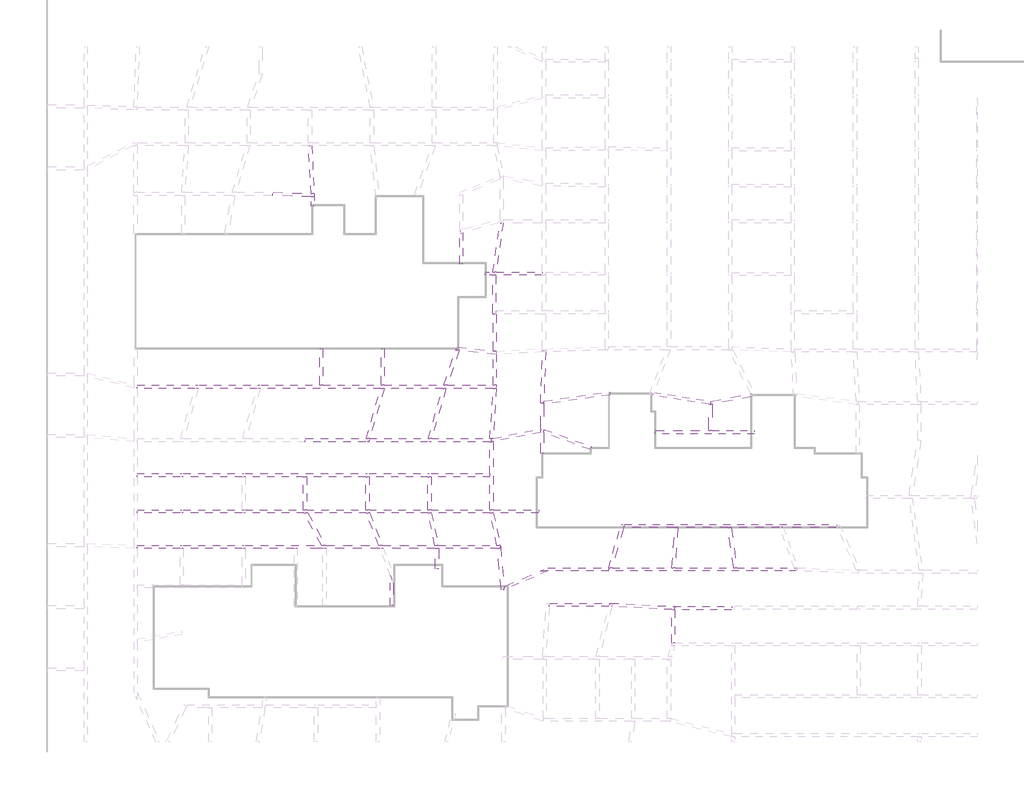
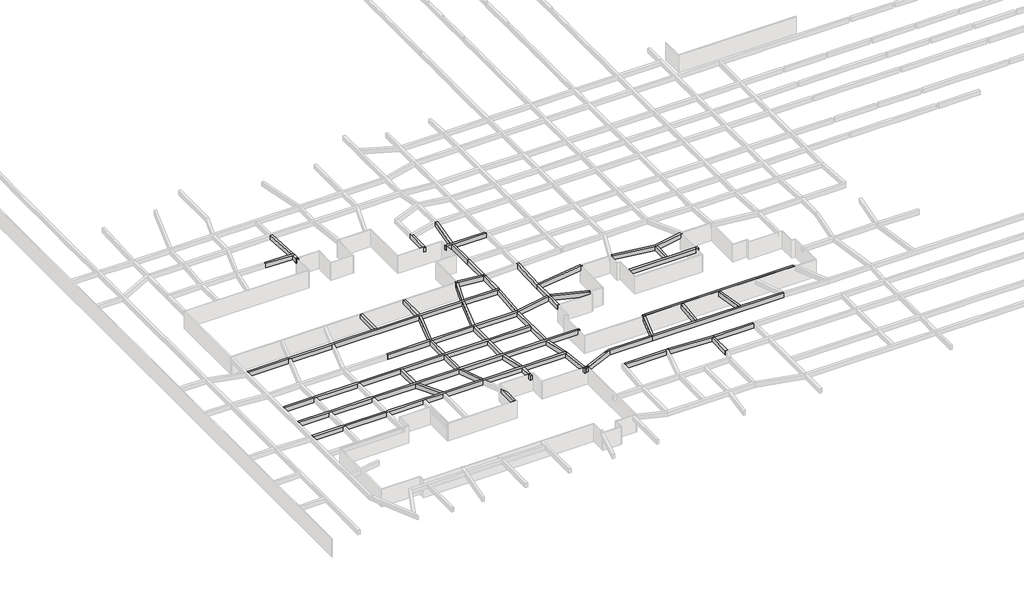
# One storey, part 19 of 45: 53 beams.
"""IFC4 building model written with IfcOpenShell, lengths in millimetres."""

from ifc_helpers import new_model, si_unit, frame, origin, place, context, project, spatial, polyline, outline, extrude, faceted_brep, element, save

model = new_model("IFC4")

# Units and contexts
model_context = context("Model", 3, world=origin())
ifc_project = project(units=[si_unit("LENGTHUNIT", "METRE", prefix="MILLI")], contexts=[model_context])

# Site, building, storey
site = spatial("IfcSite", under=ifc_project)
building = spatial("IfcBuilding", under=site)
storey = spatial("IfcBuildingStorey", under=building, Name="户型图", Elevation=0.0)

# Beams
placement = place(None, origin())
element("IfcBeam", 1, ObjectType="混凝土 - 矩形梁 : KL_beam", at=placement, inside=storey, context=model_context, shape_type="Brep", body=[
    faceted_brep([(-121416.9966498, -9324.8832397, 3300.0), (-121818.2799848, -9310.8701169, 3300.0), (-126600.5942652, -9143.8680223, 3300.0), (-126607.5762912, -9543.8680223, 3300.0), (-121807.1214928, -9711.5035977, 3300.0), (-121430.9564485, -9724.6395705, 3300.0), (-121423.7596296, -9518.5496432, 3300.0), (-126607.5762912, -9543.8680223, 2500.0), (-121807.1214928, -9711.5035977, 2500.0), (-121430.9564485, -9724.6395705, 2500.0), (-126600.5942652, -9143.8680223, 2500.0), (-121818.2799848, -9310.8701169, 2500.0), (-121416.9966498, -9324.8832397, 2500.0), (-121423.7596296, -9518.5496432, 2500.0)], [[[0, 1, 2, 3, 4, 5, 6]], [[5, 4, 3, 7, 8, 9]], [[9, 8, 7, 10, 11, 12, 13]], [[2, 1, 0, 12, 11, 10]], [[2, 10, 7, 3]], [[0, 6, 5, 9, 13, 12]]]),
])
element("IfcBeam", 2, ObjectType="混凝土 - 矩形梁 : KL_beam", at=placement, inside=storey, context=model_context, shape_type="SweptSolid", body=[
    extrude(outline(polyline([(-121416.9966498, -9324.8832397), (-121818.2799848, -9310.8701169), (-122132.953931, -3306.533538), (-121732.4049926, -3306.533538), (-121416.9966498, -9324.8832397)])), frame((0.0, 0.0, 2500.0), z_axis=(0.0, 0.0, 1.0), x_axis=(1.0, 0.0, 0.0)), (0.0, 0.0, 1.0), 800.0),
])
element("IfcBeam", 3, ObjectType="混凝土 - 矩形梁 : KL_beam", at=placement, inside=storey, context=model_context, shape_type="SweptSolid", body=[
    extrude(outline(polyline([(-121407.1214928, -10918.5496432), (-121807.1214928, -10918.5496432), (-121807.1214928, -9711.5035977), (-121430.9564485, -9724.6395705), (-121423.7596296, -9518.5496432), (-121407.1214928, -9518.5496432), (-121407.1214928, -10918.5496432)])), frame((0.0, 0.0, 2500.0), z_axis=(0.0, 0.0, 1.0), x_axis=(1.0, 0.0, 0.0)), (0.0, 0.0, 1.0), 800.0),
])
element("IfcBeam", 4, ObjectType="混凝土 - 矩形梁 : KL_beam", at=placement, inside=storey, context=model_context, shape_type="SweptSolid", body=[
    extrude(outline(polyline([(-102709.6713464, -18172.9434458), (-103109.6713464, -18172.9434458), (-103109.6713464, -13919.4780482), (-103006.1437284, -14305.8483787), (-102709.6713464, -14226.4088434), (-102709.6713464, -18172.9434458)])), frame((0.0, 0.0, 2500.0), z_axis=(0.0, 0.0, 1.0), x_axis=(1.0, 0.0, 0.0)), (0.0, 0.0, 1.0), 800.0),
])
element("IfcBeam", 5, ObjectType="混凝土 - 矩形梁 : KL_beam", at=placement, inside=storey, context=model_context, shape_type="Brep", body=[
    faceted_brep([(-99891.6040575, -19606.533538, 3300.0), (-99891.6040575, -19206.533538, 3300.0), (-99891.6040575, -19206.533538, 2500.0), (-99891.6040575, -19606.533538, 2500.0), (-98951.6884215, -19606.533538, 3300.0), (-98551.6884215, -19606.533538, 3300.0), (-92691.6701424, -19606.533538, 3300.0), (-92691.6701424, -19206.533538, 3300.0), (-98521.6747222, -19206.533538, 3300.0), (-98925.6057512, -19206.533538, 3300.0), (-92691.6701424, -19206.533538, 2500.0), (-98521.6747222, -19206.533538, 2500.0), (-98925.6057512, -19206.533538, 2500.0), (-92691.6701424, -19606.533538, 2500.0), (-98551.6884215, -19606.533538, 2500.0), (-98951.6884215, -19606.533538, 2500.0)], [[[0, 1, 2, 3]], [[1, 0, 4, 5, 6, 7, 8, 9]], [[2, 1, 9, 8, 7, 10, 11, 12]], [[3, 2, 12, 11, 10, 13, 14, 15]], [[0, 3, 15, 14, 13, 6, 5, 4]], [[7, 6, 13, 10]]]),
])
element("IfcBeam", 6, ObjectType="混凝土 - 矩形梁 : KL_beam", at=placement, inside=storey, context=model_context, shape_type="SweptSolid", body=[
    extrude(outline(polyline([(-98521.6747222, -19206.533538), (-98925.6057512, -19206.533538), (-98050.230566, -12977.9154491), (-98010.1601463, -12967.1786125), (-98010.1601463, -13006.533538), (-97650.3215471, -13006.533538), (-98521.6747222, -19206.533538)])), frame((0.0, 0.0, 2500.0), z_axis=(0.0, 0.0, 1.0), x_axis=(1.0, 0.0, 0.0)), (0.0, 0.0, 1.0), 800.0),
])
element("IfcBeam", 7, ObjectType="混凝土 - 矩形梁 : KL_beam", at=placement, inside=storey, context=model_context, shape_type="Brep", body=[
    faceted_brep([(-98951.6884215, -24466.2432363, 3300.0), (-98889.6882512, -24466.2432363, 3300.0), (-98551.6884215, -24466.2432363, 3300.0), (-98551.6884215, -24066.2432363, 3300.0), (-98551.6884215, -19606.533538, 3300.0), (-98951.6884215, -19606.533538, 3300.0), (-98951.6884215, -24466.2432363, 2500.0), (-98951.6884215, -19606.533538, 2500.0), (-98551.6884215, -24466.2432363, 2500.0), (-98889.6882512, -24466.2432363, 2500.0), (-98551.6884215, -19606.533538, 2500.0), (-98551.6884215, -24066.2432363, 2500.0)], [[[0, 1, 2, 3, 4, 5]], [[6, 0, 5, 7]], [[8, 9, 6, 7, 10, 11]], [[2, 8, 11, 10, 4, 3]], [[5, 4, 10, 7]], [[2, 1, 0, 6, 9, 8]]]),
])
element("IfcBeam", 8, ObjectType="混凝土 - 矩形梁 : KL_beam", at=placement, inside=storey, context=model_context, shape_type="Brep", body=[
    faceted_brep([(-92521.8746508, -35665.7137076, 3300.0), (-92513.6781652, -35430.9970723, 3300.0), (-92298.1056102, -29257.806784, 3300.0), (-92291.5379725, -29069.7342493, 3300.0), (-92691.5379725, -29062.7522233, 3300.0), (-92698.9743886, -29275.7033162, 3300.0), (-92921.8746508, -35658.7316817, 3300.0), (-92691.5379725, -29062.7522233, 2500.0), (-92698.9743886, -29275.7033162, 2500.0), (-92921.8746508, -35658.7316817, 2500.0), (-92291.5379725, -29069.7342493, 2500.0), (-92298.1056102, -29257.806784, 2500.0), (-92513.6781652, -35430.9970723, 2500.0), (-92521.8746508, -35665.7137076, 2500.0)], [[[0, 1, 2, 3, 4, 5, 6]], [[6, 5, 4, 7, 8, 9]], [[9, 8, 7, 10, 11, 12, 13]], [[3, 2, 1, 0, 13, 12, 11, 10]], [[3, 10, 7, 4]], [[0, 6, 9, 13]]]),
])
element("IfcBeam", 9, ObjectType="混凝土 - 矩形梁 : KL_beam", at=placement, inside=storey, context=model_context, shape_type="Brep", body=[
    faceted_brep([(-92521.8746508, -42062.2226947, 3300.0), (-92921.8746508, -42062.2226947, 3300.0), (-92921.8746508, -42062.2226947, 2500.0), (-92521.8746508, -42062.2226947, 2500.0), (-92521.8746508, -39413.7176752, 3300.0), (-92521.8746508, -38987.7193621, 3300.0), (-92521.8746508, -35836.0800422, 3300.0), (-92521.8746508, -35665.7137076, 3300.0), (-92921.8746508, -35658.7316817, 3300.0), (-92921.8746508, -38962.5802329, 3300.0), (-92921.8746508, -39370.0669109, 3300.0), (-92921.8746508, -35658.7316817, 2500.0), (-92921.8746508, -38962.5802329, 2500.0), (-92921.8746508, -39370.0669109, 2500.0), (-92521.8746508, -35665.7137076, 2500.0), (-92521.8746508, -35836.0800422, 2500.0), (-92521.8746508, -38987.7193621, 2500.0), (-92521.8746508, -39413.7176752, 2500.0)], [[[0, 1, 2, 3]], [[1, 0, 4, 5, 6, 7, 8, 9, 10]], [[2, 1, 10, 9, 8, 11, 12, 13]], [[3, 2, 13, 12, 11, 14, 15, 16, 17]], [[0, 3, 17, 16, 15, 14, 7, 6, 5, 4]], [[7, 14, 11, 8]]]),
])
element("IfcBeam", 10, ObjectType="混凝土 - 矩形梁 : KL_beam", at=placement, inside=storey, context=model_context, shape_type="Brep", body=[
    faceted_brep([(-98501.9396833, -33842.9557231, 3300.0), (-98501.9396833, -33442.9557231, 3300.0), (-98889.6882512, -33442.9557231, 3300.0), (-104704.5181871, -33442.9557231, 3300.0), (-105128.1844509, -33442.9557231, 3300.0), (-112586.1473381, -33442.9557231, 3300.0), (-112986.1473381, -33442.9557231, 3300.0), (-120315.2422867, -33442.9557231, 3300.0), (-120715.2422867, -33442.9557231, 3300.0), (-128093.2030313, -33442.9557231, 3300.0), (-128509.3228056, -33442.9557231, 3300.0), (-135893.2030313, -33442.9557231, 3300.0), (-136309.3228056, -33442.9557231, 3300.0), (-143687.6160394, -33442.9557231, 3300.0), (-143687.6160394, -33842.9557231, 3300.0), (-136424.0209599, -33842.9557231, 3300.0), (-136007.9011856, -33842.9557231, 3300.0), (-128624.0209599, -33842.9557231, 3300.0), (-128207.9011856, -33842.9557231, 3300.0), (-113051.6472072, -33842.9557231, 3300.0), (-112635.5274329, -33842.9557231, 3300.0), (-105251.569135, -33842.9557231, 3300.0), (-104835.4493606, -33842.9557231, 3300.0), (-98902.739144, -33842.9557231, 3300.0), (-98501.9396833, -33442.9557231, 2500.0), (-98889.6882512, -33442.9557231, 2500.0), (-104704.5181871, -33442.9557231, 2500.0), (-105128.1844509, -33442.9557231, 2500.0), (-112586.1473381, -33442.9557231, 2500.0), (-112986.1473381, -33442.9557231, 2500.0), (-120315.2422867, -33442.9557231, 2500.0), (-120715.2422867, -33442.9557231, 2500.0), (-128093.2030313, -33442.9557231, 2500.0), (-128509.3228056, -33442.9557231, 2500.0), (-135893.2030313, -33442.9557231, 2500.0), (-136309.3228056, -33442.9557231, 2500.0), (-143687.6160394, -33442.9557231, 2500.0), (-98501.9396833, -33842.9557231, 2500.0), (-98902.739144, -33842.9557231, 2500.0), (-104835.4493606, -33842.9557231, 2500.0), (-105251.569135, -33842.9557231, 2500.0), (-112635.5274329, -33842.9557231, 2500.0), (-113051.6472072, -33842.9557231, 2500.0), (-128207.9011856, -33842.9557231, 2500.0), (-128624.0209599, -33842.9557231, 2500.0), (-136007.9011856, -33842.9557231, 2500.0), (-136424.0209599, -33842.9557231, 2500.0), (-143687.6160394, -33842.9557231, 2500.0)], [[[0, 1, 2, 3, 4, 5, 6, 7, 8, 9, 10, 11, 12, 13, 14, 15, 16, 17, 18, 19, 20, 21, 22, 23]], [[1, 24, 25, 26, 27, 28, 29, 30, 31, 32, 33, 34, 35, 36, 13, 12, 11, 10, 9, 8, 7, 6, 5, 4, 3, 2]], [[24, 37, 38, 39, 40, 41, 42, 43, 44, 45, 46, 47, 36, 35, 34, 33, 32, 31, 30, 29, 28, 27, 26, 25]], [[37, 0, 23, 22, 21, 20, 19, 18, 17, 16, 15, 14, 47, 46, 45, 44, 43, 42, 41, 40, 39, 38]], [[14, 13, 36, 47]], [[0, 37, 24, 1]]]),
])
element("IfcBeam", 11, ObjectType="混凝土 - 矩形梁 : KL_beam", at=placement, inside=storey, context=model_context, shape_type="Brep", body=[
    faceted_brep([(-122515.2422867, -40170.1922876, 3300.0), (-122515.2422867, -40570.1922876, 3300.0), (-114915.2422867, -40570.1922876, 3300.0), (-114564.5314767, -40570.1922876, 3300.0), (-114449.8333224, -40170.1922876, 3300.0), (-114865.9530967, -40170.1922876, 3300.0), (-122515.2422867, -40570.1922876, 2500.0), (-114915.2422867, -40570.1922876, 2500.0), (-114564.5314767, -40570.1922876, 2500.0), (-122515.2422867, -40170.1922876, 2500.0), (-114865.9530967, -40170.1922876, 2500.0), (-114449.8333224, -40170.1922876, 2500.0)], [[[0, 1, 2, 3, 4, 5]], [[1, 6, 7, 8, 3, 2]], [[6, 9, 10, 11, 8, 7]], [[9, 0, 5, 4, 11, 10]], [[0, 9, 6, 1]], [[4, 3, 8, 11]]]),
])
element("IfcBeam", 12, ObjectType="混凝土 - 矩形梁 : KL_beam", at=placement, inside=storey, context=model_context, shape_type="Brep", body=[
    faceted_brep([(-99095.9844771, -40570.1922876, 3300.0), (-99134.5000963, -40170.1922876, 3300.0), (-99302.9736319, -40170.1922876, 3300.0), (-106649.7552501, -40170.1922876, 3300.0), (-107065.8750244, -40170.1922876, 3300.0), (-114449.8333224, -40170.1922876, 3300.0), (-114564.5314767, -40570.1922876, 3300.0), (-114515.2422867, -40570.1922876, 3300.0), (-107115.2422867, -40570.1922876, 3300.0), (-106715.2422867, -40570.1922876, 3300.0), (-99315.2422867, -40570.1922876, 3300.0), (-99095.9844771, -40570.1922876, 2500.0), (-114564.5314767, -40570.1922876, 2500.0), (-114515.2422867, -40570.1922876, 2500.0), (-107115.2422867, -40570.1922876, 2500.0), (-106715.2422867, -40570.1922876, 2500.0), (-99315.2422867, -40570.1922876, 2500.0), (-99134.5000963, -40170.1922876, 2500.0), (-114449.8333224, -40170.1922876, 2500.0), (-107065.8750244, -40170.1922876, 2500.0), (-106649.7552501, -40170.1922876, 2500.0), (-99302.9736319, -40170.1922876, 2500.0)], [[[0, 1, 2, 3, 4, 5, 6, 7, 8, 9, 10]], [[11, 0, 10, 9, 8, 7, 6, 12, 13, 14, 15, 16]], [[17, 11, 16, 15, 14, 13, 12, 18, 19, 20, 21]], [[1, 17, 21, 20, 19, 18, 5, 4, 3, 2]], [[1, 0, 11, 17]], [[6, 5, 18, 12]]]),
])
element("IfcBeam", 13, ObjectType="混凝土 - 矩形梁 : KL_beam", at=placement, inside=storey, context=model_context, shape_type="Brep", body=[
    faceted_brep([(-99134.5000963, -40170.1922876, 3300.0), (-99095.9844771, -40570.1922876, 3300.0), (-98915.2422867, -40535.0595648, 3300.0), (-92921.8746508, -39370.0669109, 3300.0), (-92921.8746508, -38962.5802329, 3300.0), (-98899.2820038, -40124.4705221, 3300.0), (-99095.9844771, -40570.1922876, 2500.0), (-98915.2422867, -40535.0595648, 2500.0), (-92921.8746508, -39370.0669109, 2500.0), (-99134.5000963, -40170.1922876, 2500.0), (-98899.2820038, -40124.4705221, 2500.0), (-92921.8746508, -38962.5802329, 2500.0)], [[[0, 1, 2, 3, 4, 5]], [[1, 6, 7, 8, 3, 2]], [[6, 9, 10, 11, 8, 7]], [[9, 0, 5, 4, 11, 10]], [[0, 9, 6, 1]], [[4, 3, 8, 11]]]),
])
element("IfcBeam", 14, ObjectType="混凝土 - 矩形梁 : KL_beam", at=placement, inside=storey, context=model_context, shape_type="Brep", body=[
    faceted_brep([(-143687.6160394, -44584.7380181, 3300.0), (-143687.6160394, -44984.7380181, 3300.0), (-138287.6160394, -44984.7380181, 3300.0), (-137887.6160394, -44984.7380181, 3300.0), (-130487.6160394, -44984.7380181, 3300.0), (-130087.6160394, -44984.7380181, 3300.0), (-122787.6160394, -44984.7380181, 3300.0), (-122387.6160394, -44984.7380181, 3300.0), (-114915.2422867, -44984.7380181, 3300.0), (-114515.2422867, -44984.7380181, 3300.0), (-107115.2422867, -44984.7380181, 3300.0), (-106715.2422867, -44984.7380181, 3300.0), (-99315.2422867, -44984.7380181, 3300.0), (-99315.2422867, -44584.7380181, 3300.0), (-106715.2422867, -44584.7380181, 3300.0), (-107115.2422867, -44584.7380181, 3300.0), (-114515.2422867, -44584.7380181, 3300.0), (-114915.2422867, -44584.7380181, 3300.0), (-130087.6160394, -44584.7380181, 3300.0), (-130487.6160394, -44584.7380181, 3300.0), (-137887.6160394, -44584.7380181, 3300.0), (-138287.6160394, -44584.7380181, 3300.0), (-143687.6160394, -44984.7380181, 2500.0), (-138287.6160394, -44984.7380181, 2500.0), (-137887.6160394, -44984.7380181, 2500.0), (-130487.6160394, -44984.7380181, 2500.0), (-130087.6160394, -44984.7380181, 2500.0), (-122787.6160394, -44984.7380181, 2500.0), (-122387.6160394, -44984.7380181, 2500.0), (-114915.2422867, -44984.7380181, 2500.0), (-114515.2422867, -44984.7380181, 2500.0), (-107115.2422867, -44984.7380181, 2500.0), (-106715.2422867, -44984.7380181, 2500.0), (-99315.2422867, -44984.7380181, 2500.0), (-143687.6160394, -44584.7380181, 2500.0), (-138287.6160394, -44584.7380181, 2500.0), (-137887.6160394, -44584.7380181, 2500.0), (-130487.6160394, -44584.7380181, 2500.0), (-130087.6160394, -44584.7380181, 2500.0), (-114915.2422867, -44584.7380181, 2500.0), (-114515.2422867, -44584.7380181, 2500.0), (-107115.2422867, -44584.7380181, 2500.0), (-106715.2422867, -44584.7380181, 2500.0), (-99315.2422867, -44584.7380181, 2500.0)], [[[0, 1, 2, 3, 4, 5, 6, 7, 8, 9, 10, 11, 12, 13, 14, 15, 16, 17, 18, 19, 20, 21]], [[1, 22, 23, 24, 25, 26, 27, 28, 29, 30, 31, 32, 33, 12, 11, 10, 9, 8, 7, 6, 5, 4, 3, 2]], [[22, 34, 35, 36, 37, 38, 39, 40, 41, 42, 43, 33, 32, 31, 30, 29, 28, 27, 26, 25, 24, 23]], [[34, 0, 21, 20, 19, 18, 17, 16, 15, 14, 13, 43, 42, 41, 40, 39, 38, 37, 36, 35]], [[1, 0, 34, 22]], [[13, 12, 33, 43]]]),
])
element("IfcBeam", 15, ObjectType="混凝土 - 矩形梁 : KL_beam", at=placement, inside=storey, context=model_context, shape_type="Brep", body=[
    faceted_brep([(-93173.130842, -49149.7368283, 3300.0), (-93173.130842, -49549.7368283, 3300.0), (-93173.130842, -49549.7368283, 2500.0), (-93173.130842, -49149.7368283, 2500.0), (-98915.2422867, -49149.7368283, 3300.0), (-99315.2422867, -49149.7368283, 3300.0), (-106715.2422867, -49149.7368283, 3300.0), (-107115.2422867, -49149.7368283, 3300.0), (-114515.2422867, -49149.7368283, 3300.0), (-114915.2422867, -49149.7368283, 3300.0), (-122387.6160394, -49149.7368283, 3300.0), (-122787.6160394, -49149.7368283, 3300.0), (-130087.6160394, -49149.7368283, 3300.0), (-130487.6160394, -49149.7368283, 3300.0), (-137887.6160394, -49149.7368283, 3300.0), (-138287.6160394, -49149.7368283, 3300.0), (-143687.6160394, -49149.7368283, 3300.0), (-143687.6160394, -49549.7368283, 3300.0), (-138287.6160394, -49549.7368283, 3300.0), (-137887.6160394, -49549.7368283, 3300.0), (-130487.6160394, -49549.7368283, 3300.0), (-130087.6160394, -49549.7368283, 3300.0), (-122705.4250427, -49549.7368283, 3300.0), (-122248.0834155, -49549.7368283, 3300.0), (-114852.5939636, -49549.7368283, 3300.0), (-114424.1359662, -49549.7368283, 3300.0), (-107077.1990933, -49549.7368283, 3300.0), (-106668.2628554, -49549.7368283, 3300.0), (-99277.1990933, -49549.7368283, 3300.0), (-98868.2628554, -49549.7368283, 3300.0), (-143687.6160394, -49549.7368283, 2500.0), (-138287.6160394, -49549.7368283, 2500.0), (-137887.6160394, -49549.7368283, 2500.0), (-130487.6160394, -49549.7368283, 2500.0), (-130087.6160394, -49549.7368283, 2500.0), (-122705.4250427, -49549.7368283, 2500.0), (-122248.0834155, -49549.7368283, 2500.0), (-114852.5939636, -49549.7368283, 2500.0), (-114424.1359662, -49549.7368283, 2500.0), (-107077.1990933, -49549.7368283, 2500.0), (-106668.2628554, -49549.7368283, 2500.0), (-99277.1990933, -49549.7368283, 2500.0), (-98868.2628554, -49549.7368283, 2500.0), (-143687.6160394, -49149.7368283, 2500.0), (-138287.6160394, -49149.7368283, 2500.0), (-137887.6160394, -49149.7368283, 2500.0), (-130487.6160394, -49149.7368283, 2500.0), (-130087.6160394, -49149.7368283, 2500.0), (-122787.6160394, -49149.7368283, 2500.0), (-122387.6160394, -49149.7368283, 2500.0), (-114915.2422867, -49149.7368283, 2500.0), (-114515.2422867, -49149.7368283, 2500.0), (-107115.2422867, -49149.7368283, 2500.0), (-106715.2422867, -49149.7368283, 2500.0), (-99315.2422867, -49149.7368283, 2500.0), (-98915.2422867, -49149.7368283, 2500.0)], [[[0, 1, 2, 3]], [[1, 0, 4, 5, 6, 7, 8, 9, 10, 11, 12, 13, 14, 15, 16, 17, 18, 19, 20, 21, 22, 23, 24, 25, 26, 27, 28, 29]], [[2, 1, 29, 28, 27, 26, 25, 24, 23, 22, 21, 20, 19, 18, 17, 30, 31, 32, 33, 34, 35, 36, 37, 38, 39, 40, 41, 42]], [[3, 2, 42, 41, 40, 39, 38, 37, 36, 35, 34, 33, 32, 31, 30, 43, 44, 45, 46, 47, 48, 49, 50, 51, 52, 53, 54, 55]], [[0, 3, 55, 54, 53, 52, 51, 50, 49, 48, 47, 46, 45, 44, 43, 16, 15, 14, 13, 12, 11, 10, 9, 8, 7, 6, 5, 4]], [[17, 16, 43, 30]]]),
])
element("IfcBeam", 16, ObjectType="混凝土 - 矩形梁 : KL_beam", at=placement, inside=storey, context=model_context, shape_type="Brep", body=[
    faceted_brep([(-98009.5874144, -53989.4871623, 3300.0), (-98009.5874144, -53589.4871623, 3300.0), (-98418.5236523, -53589.4871623, 3300.0), (-105809.5874144, -53589.4871623, 3300.0), (-106218.5236523, -53589.4871623, 3300.0), (-112873.4211024, -53589.4871623, 3300.0), (-113301.8790999, -53589.4871623, 3300.0), (-120008.8132398, -53589.4871623, 3300.0), (-120466.154867, -53589.4871623, 3300.0), (-130087.6160394, -53589.4871623, 3300.0), (-130487.6160394, -53589.4871623, 3300.0), (-137887.6160394, -53589.4871623, 3300.0), (-138287.6160394, -53589.4871623, 3300.0), (-143687.6160394, -53589.4871623, 3300.0), (-143687.6160394, -53989.4871623, 3300.0), (-138287.6160394, -53989.4871623, 3300.0), (-137887.6160394, -53989.4871623, 3300.0), (-130487.6160394, -53989.4871623, 3300.0), (-130087.6160394, -53989.4871623, 3300.0), (-123926.6222431, -53989.4871623, 3300.0), (-123526.6222431, -53989.4871623, 3300.0), (-120326.6222431, -53989.4871623, 3300.0), (-119926.6222431, -53989.4871623, 3300.0), (-113148.3334859, -53989.4871623, 3300.0), (-112719.8754884, -53989.4871623, 3300.0), (-106171.6416274, -53989.4871623, 3300.0), (-105771.6416274, -53989.4871623, 3300.0), (-98354.8677696, -53989.4871623, 3300.0), (-98009.5874144, -53989.4871623, 2500.0), (-143687.6160394, -53989.4871623, 2500.0), (-138287.6160394, -53989.4871623, 2500.0), (-137887.6160394, -53989.4871623, 2500.0), (-130487.6160394, -53989.4871623, 2500.0), (-130087.6160394, -53989.4871623, 2500.0), (-123926.6222431, -53989.4871623, 2500.0), (-123526.6222431, -53989.4871623, 2500.0), (-120326.6222431, -53989.4871623, 2500.0), (-119926.6222431, -53989.4871623, 2500.0), (-113148.3334859, -53989.4871623, 2500.0), (-112719.8754884, -53989.4871623, 2500.0), (-106171.6416274, -53989.4871623, 2500.0), (-105771.6416274, -53989.4871623, 2500.0), (-98354.8677696, -53989.4871623, 2500.0), (-98009.5874144, -53589.4871623, 2500.0), (-143687.6160394, -53589.4871623, 2500.0), (-138287.6160394, -53589.4871623, 2500.0), (-137887.6160394, -53589.4871623, 2500.0), (-130487.6160394, -53589.4871623, 2500.0), (-130087.6160394, -53589.4871623, 2500.0), (-120466.154867, -53589.4871623, 2500.0), (-120008.8132398, -53589.4871623, 2500.0), (-113301.8790999, -53589.4871623, 2500.0), (-112873.4211024, -53589.4871623, 2500.0), (-106218.5236523, -53589.4871623, 2500.0), (-105809.5874144, -53589.4871623, 2500.0), (-98418.5236523, -53589.4871623, 2500.0)], [[[0, 1, 2, 3, 4, 5, 6, 7, 8, 9, 10, 11, 12, 13, 14, 15, 16, 17, 18, 19, 20, 21, 22, 23, 24, 25, 26, 27]], [[28, 0, 27, 26, 25, 24, 23, 22, 21, 20, 19, 18, 17, 16, 15, 14, 29, 30, 31, 32, 33, 34, 35, 36, 37, 38, 39, 40, 41, 42]], [[43, 28, 42, 41, 40, 39, 38, 37, 36, 35, 34, 33, 32, 31, 30, 29, 44, 45, 46, 47, 48, 49, 50, 51, 52, 53, 54, 55]], [[1, 43, 55, 54, 53, 52, 51, 50, 49, 48, 47, 46, 45, 44, 13, 12, 11, 10, 9, 8, 7, 6, 5, 4, 3, 2]], [[14, 13, 44, 29]], [[1, 0, 28, 43]]]),
])
element("IfcBeam", 17, ObjectType="混凝土 - 矩形梁 : KL_beam", at=placement, inside=storey, context=model_context, shape_type="SweptSolid", body=[
    extrude(outline(polyline([(-114449.8333224, -40170.1922876), (-114865.9530967, -40170.1922876), (-113051.6472072, -33842.9557231), (-112635.5274329, -33842.9557231), (-114449.8333224, -40170.1922876)])), frame((0.0, 0.0, 2500.0), z_axis=(0.0, 0.0, 1.0), x_axis=(1.0, 0.0, 0.0)), (0.0, 0.0, 1.0), 800.0),
])
element("IfcBeam", 18, ObjectType="混凝土 - 矩形梁 : KL_beam", at=placement, inside=storey, context=model_context, shape_type="SweptSolid", body=[
    extrude(outline(polyline([(-122787.6160394, -44984.7380181), (-122387.6160394, -44984.7380181), (-122387.6160394, -49149.7368283), (-122787.6160394, -49149.7368283), (-122787.6160394, -44984.7380181)])), frame((0.0, 0.0, 2500.0), z_axis=(0.0, 0.0, 1.0), x_axis=(1.0, 0.0, 0.0)), (0.0, 0.0, 1.0), 800.0),
])
element("IfcBeam", 19, ObjectType="混凝土 - 矩形梁 : KL_beam", at=placement, inside=storey, context=model_context, shape_type="SweptSolid", body=[
    extrude(outline(polyline([(-122705.4250427, -49549.7368283), (-122248.0834155, -49549.7368283), (-120008.8132398, -53589.4871623), (-120466.154867, -53589.4871623), (-122705.4250427, -49549.7368283)])), frame((0.0, 0.0, 2500.0), z_axis=(0.0, 0.0, 1.0), x_axis=(1.0, 0.0, 0.0)), (0.0, 0.0, 1.0), 800.0),
])
element("IfcBeam", 20, ObjectType="混凝土 - 矩形梁 : KL_beam", at=placement, inside=storey, context=model_context, shape_type="Brep", body=[
    faceted_brep([(-114515.2422867, -40570.1922876, 3300.0), (-114564.5314767, -40570.1922876, 3300.0), (-114915.2422867, -40570.1922876, 3300.0), (-114915.2422867, -44584.7380181, 3300.0), (-114515.2422867, -44584.7380181, 3300.0), (-114915.2422867, -40570.1922876, 2500.0), (-114915.2422867, -44584.7380181, 2500.0), (-114564.5314767, -40570.1922876, 2500.0), (-114515.2422867, -40570.1922876, 2500.0), (-114515.2422867, -44584.7380181, 2500.0)], [[[0, 1, 2, 3, 4]], [[2, 5, 6, 3]], [[5, 7, 8, 9, 6]], [[8, 0, 4, 9]], [[5, 2, 1, 0, 8, 7]], [[4, 3, 6, 9]]]),
    faceted_brep([(-114515.2422867, -49149.7368283, 3300.0), (-114915.2422867, -49149.7368283, 3300.0), (-114915.2422867, -49149.7368283, 2500.0), (-114515.2422867, -49149.7368283, 2500.0), (-114915.2422867, -44984.7380181, 3300.0), (-114515.2422867, -44984.7380181, 3300.0), (-114515.2422867, -44984.7380181, 2500.0), (-114915.2422867, -44984.7380181, 2500.0)], [[[0, 1, 2, 3]], [[4, 5, 6, 7]], [[1, 0, 5, 4]], [[2, 1, 4, 7]], [[3, 2, 7, 6]], [[0, 3, 6, 5]]]),
])
element("IfcBeam", 21, ObjectType="混凝土 - 矩形梁 : KL_beam", at=placement, inside=storey, context=model_context, shape_type="SweptSolid", body=[
    extrude(outline(polyline([(-114852.5939636, -49549.7368283), (-114424.1359662, -49549.7368283), (-112873.4211024, -53589.4871623), (-113301.8790999, -53589.4871623), (-114852.5939636, -49549.7368283)])), frame((0.0, 0.0, 2500.0), z_axis=(0.0, 0.0, 1.0), x_axis=(1.0, 0.0, 0.0)), (0.0, 0.0, 1.0), 800.0),
])
element("IfcBeam", 22, ObjectType="混凝土 - 矩形梁 : KL_beam", at=placement, inside=storey, context=model_context, shape_type="SweptSolid", body=[
    extrude(outline(polyline([(-107115.2422867, -40570.1922876), (-106715.2422867, -40570.1922876), (-106715.2422867, -44584.7380181), (-107115.2422867, -44584.7380181), (-107115.2422867, -40570.1922876)])), frame((0.0, 0.0, 2500.0), z_axis=(0.0, 0.0, 1.0), x_axis=(1.0, 0.0, 0.0)), (0.0, 0.0, 1.0), 800.0),
    extrude(outline(polyline([(-106715.2422867, -49149.7368283), (-107115.2422867, -49149.7368283), (-107115.2422867, -44984.7380181), (-106715.2422867, -44984.7380181), (-106715.2422867, -49149.7368283)])), frame((0.0, 0.0, 2500.0), z_axis=(0.0, 0.0, 1.0), x_axis=(1.0, 0.0, 0.0)), (0.0, 0.0, 1.0), 800.0),
])
element("IfcBeam", 23, ObjectType="混凝土 - 矩形梁 : KL_beam", at=placement, inside=storey, context=model_context, shape_type="SweptSolid", body=[
    extrude(outline(polyline([(-107077.1990933, -49549.7368283), (-106668.2628554, -49549.7368283), (-105809.5874144, -53589.4871623), (-106218.5236523, -53589.4871623), (-107077.1990933, -49549.7368283)])), frame((0.0, 0.0, 2500.0), z_axis=(0.0, 0.0, 1.0), x_axis=(1.0, 0.0, 0.0)), (0.0, 0.0, 1.0), 800.0),
])
element("IfcBeam", 24, ObjectType="混凝土 - 矩形梁 : KL_beam", at=placement, inside=storey, context=model_context, shape_type="Brep", body=[
    faceted_brep([(-99095.9844771, -40570.1922876, 3300.0), (-99315.2422867, -40570.1922876, 3300.0), (-99315.2422867, -44584.7380181, 3300.0), (-99315.2422867, -44984.7380181, 3300.0), (-99315.2422867, -49149.7368283, 3300.0), (-98915.2422867, -49149.7368283, 3300.0), (-98915.2422867, -40535.0595648, 3300.0), (-99315.2422867, -40570.1922876, 2500.0), (-99315.2422867, -44584.7380181, 2500.0), (-99315.2422867, -44984.7380181, 2500.0), (-99315.2422867, -49149.7368283, 2500.0), (-99095.9844771, -40570.1922876, 2500.0), (-98915.2422867, -40535.0595648, 2500.0), (-98915.2422867, -49149.7368283, 2500.0)], [[[0, 1, 2, 3, 4, 5, 6]], [[1, 7, 8, 9, 10, 4, 3, 2]], [[7, 11, 12, 13, 10, 9, 8]], [[12, 6, 5, 13]], [[1, 0, 11, 7]], [[0, 6, 12, 11]], [[5, 4, 10, 13]]]),
])
element("IfcBeam", 25, ObjectType="混凝土 - 矩形梁 : KL_beam", at=placement, inside=storey, context=model_context, shape_type="SweptSolid", body=[
    extrude(outline(polyline([(-98009.5874144, -53589.4871623), (-98418.5236523, -53589.4871623), (-99277.1990933, -49549.7368283), (-98868.2628554, -49549.7368283), (-98009.5874144, -53589.4871623)])), frame((0.0, 0.0, 2500.0), z_axis=(0.0, 0.0, 1.0), x_axis=(1.0, 0.0, 0.0)), (0.0, 0.0, 1.0), 800.0),
])
element("IfcBeam", 26, ObjectType="混凝土 - 矩形梁 : KL_beam", at=placement, inside=storey, context=model_context, shape_type="Brep", body=[
    faceted_brep([(-97497.8255668, -59196.0390677, 3300.0), (-97534.4934161, -58776.9236321, 3300.0), (-97973.4688225, -53759.4117772, 3300.0), (-98009.5874144, -53589.4871623, 3300.0), (-98009.5874144, -53989.4871623, 3300.0), (-98354.8677696, -53989.4871623, 3300.0), (-97896.303446, -59230.9013648, 3300.0), (-97896.303446, -59230.9013648, 2500.0), (-98354.8677696, -53989.4871623, 2500.0), (-97973.4688225, -53759.4117772, 2500.0), (-97534.4934161, -58776.9236321, 2500.0), (-97497.8255668, -59196.0390677, 2500.0), (-98009.5874144, -53989.4871623, 2500.0), (-98009.5874144, -53589.4871623, 2500.0)], [[[0, 1, 2, 3, 4, 5, 6]], [[7, 6, 5, 8]], [[9, 10, 11, 7, 8, 12, 13]], [[2, 1, 0, 11, 10, 9]], [[3, 2, 9, 13]], [[4, 12, 8, 5]], [[12, 4, 3, 13]], [[0, 6, 7, 11]]]),
])
element("IfcBeam", 27, ObjectType="混凝土 - 矩形梁 : KL_beam", at=placement, inside=storey, context=model_context, shape_type="SweptSolid", body=[
    extrude(outline(polyline([(-105771.6416274, -56588.7580318), (-106171.6416274, -56588.7580318), (-106171.6416274, -53989.4871623), (-105771.6416274, -53989.4871623), (-105771.6416274, -56588.7580318)])), frame((0.0, 0.0, 2500.0), z_axis=(0.0, 0.0, 1.0), x_axis=(1.0, 0.0, 0.0)), (0.0, 0.0, 1.0), 800.0),
])
element("IfcBeam", 28, ObjectType="混凝土 - 矩形梁 : KL_beam", at=placement, inside=storey, context=model_context, shape_type="SweptSolid", body=[
    extrude(outline(polyline([(-111449.0790859, -61137.092783), (-111849.0790859, -61137.092783), (-111849.0790859, -57374.1605919), (-111449.0790859, -58416.1962178), (-111449.0790859, -61137.092783)])), frame((0.0, 0.0, 2500.0), z_axis=(0.0, 0.0, 1.0), x_axis=(1.0, 0.0, 0.0)), (0.0, 0.0, 1.0), 800.0),
])
element("IfcBeam", 29, ObjectType="混凝土 - 矩形梁 : KL_beam", at=placement, inside=storey, context=model_context, shape_type="SweptSolid", body=[
    extrude(outline(polyline([(-105251.569135, -33842.9557231), (-104835.4493606, -33842.9557231), (-106649.7552501, -40170.1922876), (-107065.8750244, -40170.1922876), (-105251.569135, -33842.9557231)])), frame((0.0, 0.0, 2500.0), z_axis=(0.0, 0.0, 1.0), x_axis=(1.0, 0.0, 0.0)), (0.0, 0.0, 1.0), 800.0),
])
element("IfcBeam", 30, ObjectType="混凝土 - 矩形梁 : KL_beam", at=placement, inside=storey, context=model_context, shape_type="Brep", body=[
    faceted_brep([(-98476.6373585, -33442.9557231, 3300.0), (-98489.6882512, -33442.9557231, 3300.0), (-98501.9396833, -33442.9557231, 3300.0), (-98501.9396833, -33842.9557231, 3300.0), (-98476.6373585, -33442.9557231, 2500.0), (-98899.2820038, -40124.4705221, 3300.0), (-98899.2820038, -40124.4705221, 2500.0), (-98501.9396833, -33842.9557231, 2500.0), (-98501.9396833, -33442.9557231, 2500.0), (-98489.6882512, -33442.9557231, 2500.0), (-98902.739144, -33842.9557231, 3300.0), (-98902.739144, -33842.9557231, 2500.0), (-99302.9736319, -40170.1922876, 2500.0), (-99302.9736319, -40170.1922876, 3300.0), (-99134.5000963, -40170.1922876, 3300.0), (-99134.5000963, -40170.1922876, 2500.0)], [[[0, 1, 2, 3]], [[4, 0, 3, 5, 6, 7]], [[8, 9, 4, 7]], [[10, 11, 12, 13]], [[0, 4, 9, 8, 2, 1]], [[3, 7, 11, 10]], [[7, 3, 2, 8]], [[3, 10, 13, 14, 5]], [[11, 7, 6, 15, 12]], [[15, 14, 13, 12]], [[14, 15, 6, 5]]]),
])
element("IfcBeam", 31, ObjectType="混凝土 - 矩形梁 : KL_beam", at=placement, inside=storey, context=model_context, shape_type="Brep", body=[
    faceted_brep([(-98489.6882512, -29133.8276372, 3300.0), (-98682.929173, -29142.4547556, 3300.0), (-98889.6882512, -29151.6853834, 3300.0), (-98889.6882512, -33442.9557231, 3300.0), (-98501.9396833, -33442.9557231, 3300.0), (-98489.6882512, -33442.9557231, 3300.0), (-98489.6882512, -29534.2260627, 3300.0), (-98489.6882512, -29133.8276372, 2500.0), (-98489.6882512, -33442.9557231, 2500.0), (-98489.6882512, -29534.2260627, 2500.0), (-98889.6882512, -29151.6853834, 2500.0), (-98682.929173, -29142.4547556, 2500.0), (-98501.9396833, -33442.9557231, 2500.0), (-98889.6882512, -33442.9557231, 2500.0)], [[[0, 1, 2, 3, 4, 5, 6]], [[7, 0, 6, 5, 8, 9]], [[10, 11, 7, 9, 8, 12, 13]], [[13, 3, 2, 10]], [[3, 13, 12, 8, 5, 4]], [[2, 1, 0, 7, 11, 10]]]),
])
element("IfcBeam", 32, ObjectType="混凝土 - 矩形梁 : KL_beam", at=placement, inside=storey, context=model_context, shape_type="SweptSolid", body=[
    extrude(outline(polyline([(-84233.4038798, -34267.2804127), (-84177.7346394, -34663.3876402), (-92521.8746508, -35836.0800422), (-92521.8746508, -35665.7137076), (-92513.6781652, -35430.9970723), (-84233.4038798, -34267.2804127)])), frame((0.0, 0.0, 2500.0), z_axis=(0.0, 0.0, 1.0), x_axis=(1.0, 0.0, 0.0)), (0.0, 0.0, 1.0), 800.0),
])
element("IfcBeam", 33, ObjectType="混凝土 - 矩形梁 : KL_beam", at=placement, inside=storey, context=model_context, shape_type="SweptSolid", body=[
    extrude(outline(polyline([(-86553.285111, -41174.3422368), (-86690.8837939, -41549.9305786), (-92521.8746508, -39413.7176752), (-92521.8746508, -38987.7193621), (-86553.285111, -41174.3422368)])), frame((0.0, 0.0, 2500.0), z_axis=(0.0, 0.0, 1.0), x_axis=(1.0, 0.0, 0.0)), (0.0, 0.0, 1.0), 800.0),
])
element("IfcBeam", 34, ObjectType="混凝土 - 矩形梁 : KL_beam", at=placement, inside=storey, context=model_context, shape_type="Brep", body=[
    faceted_brep([(-60705.9072961, -56839.7832418, 3300.0), (-60698.9252702, -56439.7832418, 3300.0), (-60988.0458845, -56439.7832418, 3300.0), (-68227.1784385, -56439.7832418, 3300.0), (-68631.2189166, -56439.7832418, 3300.0), (-76006.2262167, -56439.7832418, 3300.0), (-76407.2029759, -56439.7832418, 3300.0), (-83937.0073188, -56439.7832418, 3300.0), (-84353.1270932, -56439.7832418, 3300.0), (-84353.1270932, -56839.7832418, 3300.0), (-60705.9072961, -56839.7832418, 2500.0), (-84353.1270932, -56839.7832418, 2500.0), (-60698.9252702, -56439.7832418, 2500.0), (-84353.1270932, -56439.7832418, 2500.0), (-83937.0073188, -56439.7832418, 2500.0), (-76407.2029759, -56439.7832418, 2500.0), (-76006.2262167, -56439.7832418, 2500.0), (-68631.2189166, -56439.7832418, 2500.0), (-68227.1784385, -56439.7832418, 2500.0), (-60988.0458845, -56439.7832418, 2500.0)], [[[0, 1, 2, 3, 4, 5, 6, 7, 8, 9]], [[10, 0, 9, 11]], [[12, 10, 11, 13, 14, 15, 16, 17, 18, 19]], [[1, 12, 19, 18, 17, 16, 15, 14, 13, 8, 7, 6, 5, 4, 3, 2]], [[1, 0, 10, 12]], [[8, 13, 11, 9]]]),
])
element("IfcBeam", 35, ObjectType="混凝土 - 矩形梁 : KL_beam", at=placement, inside=storey, context=model_context, shape_type="SweptSolid", body=[
    extrude(outline(polyline([(-91804.5472216, -60887.8093836), (-84266.1304086, -60887.8093836), (-84365.8616097, -61287.8093836), (-91832.5179464, -61287.8093836), (-91804.5472216, -60887.8093836)])), frame((0.0, 0.0, 2500.0), z_axis=(0.0, 0.0, 1.0), x_axis=(1.0, 0.0, 0.0)), (0.0, 0.0, 1.0), 800.0),
])
element("IfcBeam", 36, ObjectType="混凝土 - 矩形梁 : KL_beam", at=placement, inside=storey, context=model_context, shape_type="Brep", body=[
    faceted_brep([(-84104.636099, -60887.8093836, 3300.0), (-84266.1304086, -60887.8093836, 3300.0), (-83878.0121181, -60984.5781419, 3300.0), (-83953.616158, -61287.8093836, 3300.0), (-83955.6991422, -61296.1637772, 3300.0), (-76420.6999587, -61691.0563513, 3300.0), (-76020.6999587, -61712.019463, 3300.0), (-76020.6999587, -61701.2648408, 3300.0), (-76020.6999587, -61311.4705246, 3300.0), (-76215.436006, -61301.2648408, 3300.0), (-83955.6991422, -61296.1637772, 2500.0), (-76420.6999587, -61691.0563513, 2500.0), (-76020.6999587, -61712.019463, 2500.0), (-84266.1304086, -60887.8093836, 2500.0), (-84104.636099, -60887.8093836, 2500.0), (-76215.436006, -61301.2648408, 2500.0), (-76020.6999587, -61311.4705246, 2500.0), (-76020.6999587, -61701.2648408, 2500.0), (-83953.616158, -61287.8093836, 2500.0), (-83878.0121181, -60984.5781419, 2500.0)], [[[0, 1, 2, 3, 4, 5, 6, 7, 8, 9]], [[4, 10, 11, 12, 6, 5]], [[13, 14, 15, 16, 17, 12, 11, 10, 18, 19]], [[14, 0, 9, 8, 16, 15]], [[1, 0, 14, 13]], [[2, 19, 18, 10, 4, 3]], [[19, 2, 1, 13]], [[8, 7, 6, 12, 17, 16]]]),
])
element("IfcBeam", 37, ObjectType="混凝土 - 矩形梁 : KL_beam", at=placement, inside=storey, context=model_context, shape_type="SweptSolid", body=[
    extrude(outline(polyline([(-76020.6999587, -65862.2662437), (-76420.6999587, -65862.2662437), (-76420.6999587, -61691.0563513), (-76020.6999587, -61712.019463), (-76020.6999587, -65862.2662437)])), frame((0.0, 0.0, 2500.0), z_axis=(0.0, 0.0, 1.0), x_axis=(1.0, 0.0, 0.0)), (0.0, 0.0, 1.0), 800.0),
])
element("IfcBeam", 38, ObjectType="混凝土 - 矩形梁 : KL_beam", at=placement, inside=storey, context=model_context, shape_type="SweptSolid", body=[
    extrude(outline(polyline([(-68900.6999587, -61301.2648408), (-68900.6999587, -61701.2648408), (-76020.6999587, -61701.2648408), (-76020.6999587, -61311.4705246), (-76215.436006, -61301.2648408), (-68900.6999587, -61301.2648408)])), frame((0.0, 0.0, 2500.0), z_axis=(0.0, 0.0, 1.0), x_axis=(1.0, 0.0, 0.0)), (0.0, 0.0, 1.0), 800.0),
])
element("IfcBeam", 39, ObjectType="混凝土 - 矩形梁 : KL_beam", at=placement, inside=storey, context=model_context, shape_type="Brep", body=[
    faceted_brep([(-78831.4278308, -34714.7552327, 3300.0), (-71745.5456794, -35837.0487115, 3300.0), (-71542.0196166, -35869.284073, 3300.0), (-71549.1082718, -35463.17529, 3300.0), (-78684.8781897, -34332.9803653, 3300.0), (-78831.4278308, -34714.7552327, 2500.0), (-71745.5456794, -35837.0487115, 2500.0), (-71542.0196166, -35869.284073, 2500.0), (-78684.8781897, -34332.9803653, 2500.0), (-71549.1082718, -35463.17529, 2500.0)], [[[0, 1, 2, 3, 4]], [[2, 1, 0, 5, 6, 7]], [[7, 6, 5, 8, 9]], [[3, 9, 8, 4]], [[0, 4, 8, 5]], [[3, 2, 7, 9]]]),
])
element("IfcBeam", 40, ObjectType="混凝土 - 矩形梁 : KL_beam", at=placement, inside=storey, context=model_context, shape_type="Brep", body=[
    faceted_brep([(-71542.0196166, -35869.284073, 3300.0), (-71345.5456794, -35831.0934084, 3300.0), (-66326.6265104, -34855.5143488, 3300.0), (-66508.160593, -34483.3143219, 3300.0), (-71549.1082718, -35463.17529, 3300.0), (-71542.0196166, -35869.284073, 2500.0), (-71345.5456794, -35831.0934084, 2500.0), (-66326.6265104, -34855.5143488, 2500.0), (-71549.1082718, -35463.17529, 2500.0), (-66508.160593, -34483.3143219, 2500.0)], [[[0, 1, 2, 3, 4]], [[2, 1, 0, 5, 6, 7]], [[7, 6, 5, 8, 9]], [[8, 4, 3, 9]], [[4, 8, 5, 0]], [[3, 2, 7, 9]]]),
])
element("IfcBeam", 41, ObjectType="混凝土 - 矩形梁 : KL_beam", at=placement, inside=storey, context=model_context, shape_type="SweptSolid", body=[
    extrude(outline(polyline([(-71542.0196166, -35869.284073), (-71345.5456794, -35831.0934084), (-71345.5456794, -39162.7742653), (-71745.5456794, -39162.7742653), (-71745.5456794, -35837.0487115), (-71542.0196166, -35869.284073)])), frame((0.0, 0.0, 2500.0), z_axis=(0.0, 0.0, 1.0), x_axis=(1.0, 0.0, 0.0)), (0.0, 0.0, 1.0), 800.0),
])
element("IfcBeam", 42, ObjectType="混凝土 - 矩形梁 : KL_beam", at=placement, inside=storey, context=model_context, shape_type="Brep", body=[
    faceted_brep([(-66045.5182206, -39162.7742653, 3300.0), (-66045.5182206, -39562.7742653, 3300.0), (-66045.5182206, -39562.7742653, 2500.0), (-66045.5182206, -39162.7742653, 2500.0), (-78524.5182206, -39162.7742653, 3300.0), (-78524.5182206, -39162.7742653, 2500.0), (-78524.5182206, -39562.7742653, 2500.0), (-78524.5182206, -39562.7742653, 3300.0), (-71345.5456794, -39162.7742653, 3300.0), (-71745.5456794, -39162.7742653, 3300.0), (-71745.5456794, -39162.7742653, 2500.0), (-71345.5456794, -39162.7742653, 2500.0)], [[[0, 1, 2, 3]], [[4, 5, 6, 7]], [[1, 0, 8, 9, 4, 7]], [[2, 1, 7, 6]], [[3, 2, 6, 5, 10, 11]], [[0, 3, 11, 10, 5, 4, 9, 8]]]),
])
element("IfcBeam", 43, ObjectType="混凝土 - 矩形梁 : KL_beam", at=placement, inside=storey, context=model_context, shape_type="Brep", body=[
    faceted_brep([(-92043.2067826, -56439.7832418, 3300.0), (-92983.0367828, -56839.7832418, 3300.0), (-91961.6257837, -56839.7832418, 3300.0), (-84353.1270932, -56839.7832418, 3300.0), (-84353.1270932, -56439.7832418, 3300.0), (-92043.2067826, -56439.7832418, 2500.0), (-84353.1270932, -56439.7832418, 2500.0), (-92983.0367828, -56839.7832418, 2500.0), (-84353.1270932, -56839.7832418, 2500.0), (-91961.6257837, -56839.7832418, 2500.0)], [[[0, 1, 2, 3, 4]], [[5, 0, 4, 6]], [[7, 5, 6, 8, 9]], [[1, 7, 9, 8, 3, 2]], [[4, 3, 8, 6]], [[1, 0, 5, 7]]]),
])
element("IfcBeam", 44, ObjectType="混凝土 - 矩形梁 : KL_beam", at=placement, inside=storey, context=model_context, shape_type="SweptSolid", body=[
    extrude(outline(polyline([(-97497.8255668, -59196.0390677), (-97534.4934161, -58776.9236321), (-92983.0367828, -56839.7832418), (-91961.6257837, -56839.7832418), (-97497.8255668, -59196.0390677)])), frame((0.0, 0.0, 2500.0), z_axis=(0.0, 0.0, 1.0), x_axis=(1.0, 0.0, 0.0)), (0.0, 0.0, 1.0), 800.0),
])
element("IfcBeam", 45, ObjectType="混凝土 - 矩形梁 : KL_beam", at=placement, inside=storey, context=model_context, shape_type="Brep", body=[
    faceted_brep([(-82365.8743907, -50960.5915749, 3300.0), (-82781.994165, -50960.5915749, 3300.0), (-84353.1270932, -56439.7832418, 3300.0), (-83937.0073188, -56439.7832418, 3300.0), (-82480.572545, -51360.5915749, 3300.0), (-82365.8743907, -50960.5915749, 2500.0), (-83937.0073188, -56439.7832418, 2500.0), (-82480.572545, -51360.5915749, 2500.0), (-82781.994165, -50960.5915749, 2500.0), (-84353.1270932, -56439.7832418, 2500.0)], [[[0, 1, 2, 3, 4]], [[5, 0, 4, 3, 6, 7]], [[8, 5, 7, 6, 9]], [[1, 8, 9, 2]], [[3, 2, 9, 6]], [[1, 0, 5, 8]]]),
])
element("IfcBeam", 46, ObjectType="混凝土 - 矩形梁 : KL_beam", at=placement, inside=storey, context=model_context, shape_type="SweptSolid", body=[
    extrude(outline(polyline([(-76006.2262167, -56439.7832418), (-76407.2029759, -56439.7832418), (-76052.0312954, -51360.5915749), (-75651.0545362, -51360.5915749), (-76006.2262167, -56439.7832418)])), frame((0.0, 0.0, 2500.0), z_axis=(0.0, 0.0, 1.0), x_axis=(1.0, 0.0, 0.0)), (0.0, 0.0, 1.0), 800.0),
])
element("IfcBeam", 47, ObjectType="混凝土 - 矩形梁 : KL_beam", at=placement, inside=storey, context=model_context, shape_type="SweptSolid", body=[
    extrude(outline(polyline([(-68227.1784385, -56439.7832418), (-68631.2189166, -56439.7832418), (-69354.9711926, -51360.5915749), (-68950.9307146, -51360.5915749), (-68227.1784385, -56439.7832418)])), frame((0.0, 0.0, 2500.0), z_axis=(0.0, 0.0, 1.0), x_axis=(1.0, 0.0, 0.0)), (0.0, 0.0, 1.0), 800.0),
])
element("IfcBeam", 48, ObjectType="混凝土 - 矩形梁 : KL_beam", at=placement, inside=storey, context=model_context, shape_type="Brep", body=[
    faceted_brep([(-82365.8743907, -50960.5915749, 3300.0), (-82480.572545, -51360.5915749, 3300.0), (-76052.0312954, -51360.5915749, 3300.0), (-75651.0545362, -51360.5915749, 3300.0), (-69354.9711926, -51360.5915749, 3300.0), (-68950.9307146, -51360.5915749, 3300.0), (-62836.7204654, -51360.5915749, 3300.0), (-62411.0493564, -51360.5915749, 3300.0), (-55577.7545645, -51360.5915749, 3300.0), (-55755.8460387, -50960.5915749, 3300.0), (-82480.572545, -51360.5915749, 2500.0), (-76052.0312954, -51360.5915749, 2500.0), (-75651.0545362, -51360.5915749, 2500.0), (-69354.9711926, -51360.5915749, 2500.0), (-68950.9307146, -51360.5915749, 2500.0), (-62836.7204654, -51360.5915749, 2500.0), (-62411.0493564, -51360.5915749, 2500.0), (-55577.7545645, -51360.5915749, 2500.0), (-82365.8743907, -50960.5915749, 2500.0), (-55755.8460387, -50960.5915749, 2500.0)], [[[0, 1, 2, 3, 4, 5, 6, 7, 8, 9]], [[1, 10, 11, 12, 13, 14, 15, 16, 17, 8, 7, 6, 5, 4, 3, 2]], [[10, 18, 19, 17, 16, 15, 14, 13, 12, 11]], [[18, 0, 9, 19]], [[1, 0, 18, 10]], [[9, 8, 17, 19]]]),
])
element("IfcBeam", 49, ObjectType="混凝土 - 矩形梁 : KL_beam", at=placement, inside=storey, context=model_context, shape_type="Brep", body=[
    faceted_brep([(-103440.3561476, -28607.3846948, 3300.0), (-103575.5469228, -28994.7016954, 3300.0), (-103167.8843395, -29040.5516989, 3300.0), (-98489.6882512, -29566.7106244, 3300.0), (-98489.6882512, -29164.1886534, 3300.0), (-98682.929173, -29142.4547556, 3300.0), (-98889.6882512, -29119.2004643, 3300.0), (-103440.3561476, -28607.3846948, 2500.0), (-98489.6882512, -29164.1886534, 2500.0), (-98682.929173, -29142.4547556, 2500.0), (-98889.6882512, -29119.2004643, 2500.0), (-103575.5469228, -28994.7016954, 2500.0), (-98489.6882512, -29566.7106244, 2500.0), (-103167.8843395, -29040.5516989, 2500.0)], [[[0, 1, 2, 3, 4, 5, 6]], [[7, 0, 6, 5, 4, 8, 9, 10]], [[11, 7, 10, 9, 8, 12, 13]], [[1, 11, 13, 12, 3, 2]], [[4, 3, 12, 8]], [[1, 0, 7, 11]]]),
])
element("IfcBeam", 50, ObjectType="混凝土 - 矩形梁 : KL_beam", at=placement, inside=storey, context=model_context, shape_type="SweptSolid", body=[
    extrude(outline(polyline([(-112986.1473381, -28823.9118727), (-112586.1473381, -28823.9118727), (-112586.1473381, -33442.9557231), (-112986.1473381, -33442.9557231), (-112986.1473381, -28823.9118727)])), frame((0.0, 0.0, 2500.0), z_axis=(0.0, 0.0, 1.0), x_axis=(1.0, 0.0, 0.0)), (0.0, 0.0, 1.0), 800.0),
])
element("IfcBeam", 51, ObjectType="混凝土 - 矩形梁 : KL_beam", at=placement, inside=storey, context=model_context, shape_type="SweptSolid", body=[
    extrude(outline(polyline([(-120715.2422867, -28823.9118727), (-120315.2422867, -28823.9118727), (-120315.2422867, -33442.9557231), (-120715.2422867, -33442.9557231), (-120715.2422867, -28823.9118727)])), frame((0.0, 0.0, 2500.0), z_axis=(0.0, 0.0, 1.0), x_axis=(1.0, 0.0, 0.0)), (0.0, 0.0, 1.0), 800.0),
])
element("IfcBeam", 52, ObjectType="混凝土 - 矩形梁 : KL_beam", at=placement, inside=storey, context=model_context, shape_type="SweptSolid", body=[
    extrude(outline(polyline([(-104704.5181871, -33442.9557231), (-105128.1844509, -33442.9557231), (-103575.5469228, -28994.7016954), (-103167.8843395, -29040.5516989), (-104704.5181871, -33442.9557231)])), frame((0.0, 0.0, 2500.0), z_axis=(0.0, 0.0, 1.0), x_axis=(1.0, 0.0, 0.0)), (0.0, 0.0, 1.0), 800.0),
])
element("IfcBeam", 53, ObjectType="混凝土 - 矩形梁 : KL_beam", at=placement, inside=storey, context=model_context, shape_type="Brep", body=[
    faceted_brep([(-98489.6882512, -24466.2432363, 3300.0), (-98551.6884215, -24466.2432363, 3300.0), (-98889.6882512, -24466.2432363, 3300.0), (-98889.6882512, -29119.2004643, 3300.0), (-98682.929173, -29142.4547556, 3300.0), (-98489.6882512, -29133.8276372, 3300.0), (-98489.6882512, -24466.2432363, 2500.0), (-98489.6882512, -29133.8276372, 2500.0), (-98889.6882512, -24466.2432363, 2500.0), (-98551.6884215, -24466.2432363, 2500.0), (-98682.929173, -29142.4547556, 2500.0), (-98889.6882512, -29119.2004643, 2500.0)], [[[0, 1, 2, 3, 4, 5]], [[6, 0, 5, 7]], [[8, 9, 6, 7, 10, 11]], [[2, 8, 11, 3]], [[8, 2, 1, 0, 6, 9]], [[7, 5, 4, 10]], [[4, 3, 11, 10]]]),
])

save(model, "model.ifc")

# Revit data of these elements
# Type "混凝土 - 矩形梁 : KL_beam"
#   Length [instance default] = 1524 mm
#   b = 400 mm
#   h = 800 mm
#   Structural Material [instance default] = 混凝土 - 现场浇注混凝土
#   Assembly Code = ""
# Elements 1, 2, 3, 4, 5, 6, 7, 8, 9, 10, 11, 12, 13, 14, 15, 16, 17, 18, 19, 20, 21, 22, 23, 24, 25, 26, 27, 28, 29, 30, 31, 32, 33, 34, 35, 36, 37, 38, 39, 40, 41, 42, 43, 44, 45, 46, 47, 48, 49, 50, 51, 52, 53 (IfcBeam, "混凝土 - 矩形梁 : KL_beam")
#   Comments = ""
#   Structural Material = none
#   Phase Created = 新构造
# Materials
#   "混凝土 - 现场浇注混凝土": class "混凝土", colour RGB 192 192 192, transparency 0
